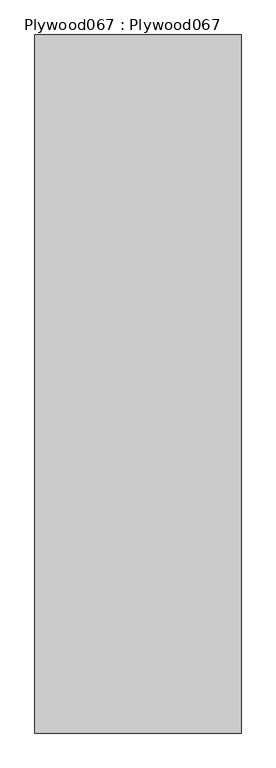
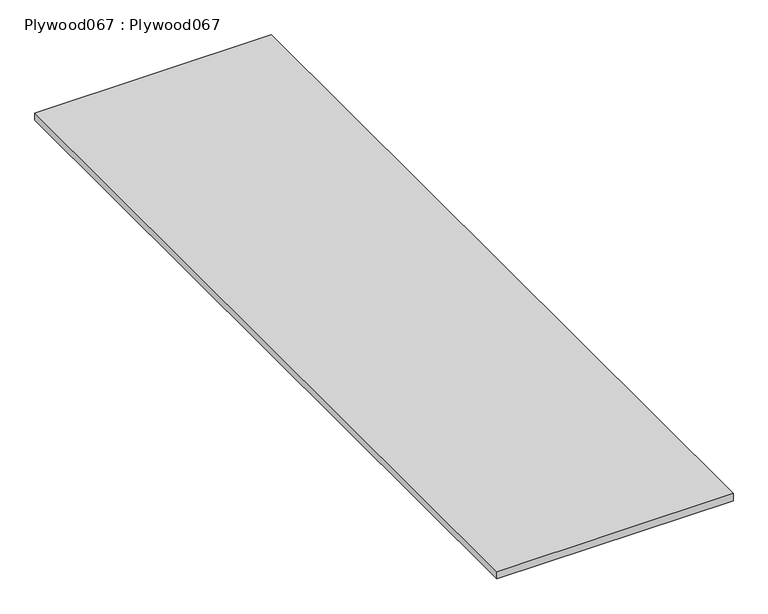
"""IFC4 building model written with IfcOpenShell, lengths in millimetres: proxy geometry, Plywood067 : Plywood067."""

from ifc_helpers import new_model, si_unit, frame, origin, place, context, project, spatial, polyline, outline, extrude, source, transform, mapped, element, save


def plywood067_plywood067_cead1058(model_context):
    return source(origin(), model_context, "Body", "SweptSolid", [
        extrude(outline(polyline([(-9298.3737014, 7982.1531721), (-9888.9237014, 7982.1531721), (-9888.9237014, 9982.1531721), (-9298.3737014, 9982.1531721), (-9298.3737014, 7982.1531721)])), frame((0.0, 0.0, 39560.2460083), z_axis=(0.0, 0.0, 1.0), x_axis=(1.0, 0.0, 0.0)), (0.0, 0.0, 1.0), 19.05),
    ])


if __name__ == "__main__":
    model = new_model("IFC4")
    model_context = context("Model", 3, world=origin())
    ifc_project = project(units=[si_unit("LENGTHUNIT", "METRE", prefix="MILLI")], contexts=[model_context])
    site = spatial("IfcSite", under=ifc_project)
    building = spatial("IfcBuilding", under=site)
    placement = place(None, origin())
    plywood067_plywood067_shape = plywood067_plywood067_cead1058(model_context)
    element("IfcBuildingElementProxy", 1, Name="Plywood067 : Plywood067", ObjectType="Plywood067 : Plywood067", at=placement, inside=building, context=model_context, shape_type="MappedRepresentation", body=[
        mapped(plywood067_plywood067_shape, transform((0.0, 0.0, 0.0), x_axis=(1.0, 0.0, 0.0), y_axis=(0.0, 1.0, 0.0), z_axis=(0.0, 0.0, 1.0))),
    ])
    save(model, "model.ifc")

# Revit data of these elements
# Type "Plywood067 : Plywood067"
#   NameOverride = "Plywood067"
# Element 1 (IfcBuildingElementProxy, "Plywood067 : Plywood067")
#   Materials on its faces: "CDX PLYWOOD - SEE STRUCTURAL DWGS"
# Materials
#   "CDX PLYWOOD - SEE STRUCTURAL DWGS": class "Unassigned", colour RGB 177 130 114, transparency 0, Cost = 0
